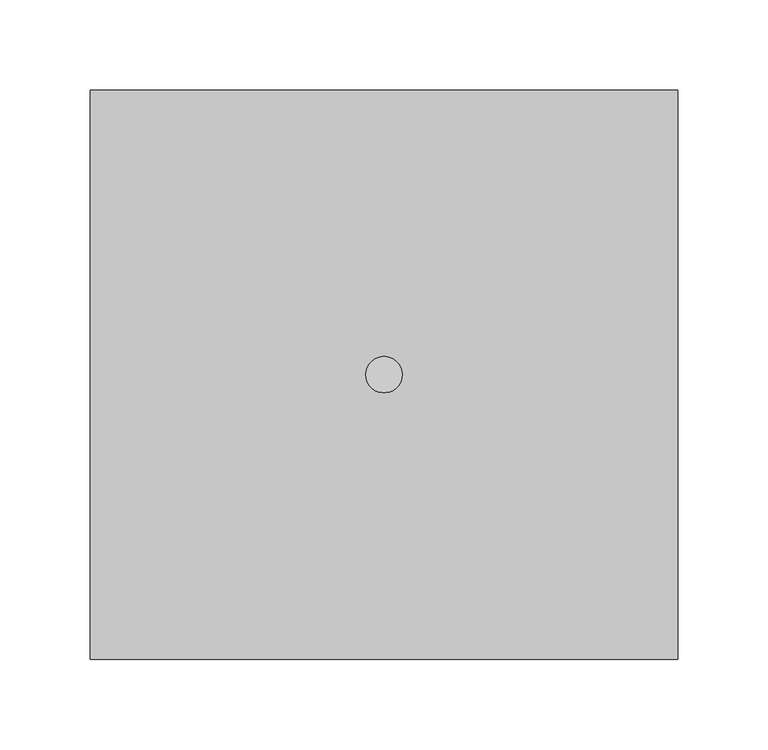
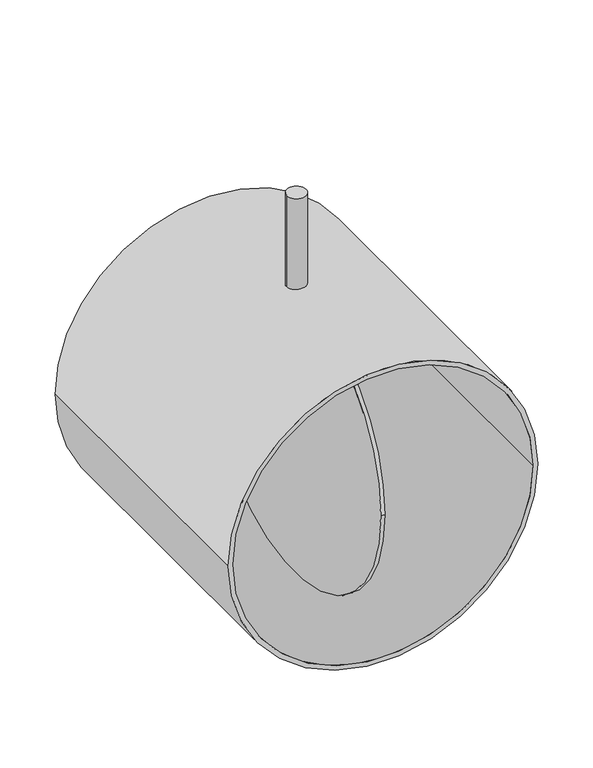
"""IFC4 building model written with IfcOpenShell, lengths in millimetres: proxy geometry, Заслонка регулирующая DFGR : DFGR 315."""

from ifc_helpers import new_model, si_unit, point, frame, origin, origin_2d, place, context, project, spatial, circle_curve, trimmed, segment, composite_curve, outline, extrude, source, transform, mapped, element, save


def mechanical_equipment_7cf25c75(model_context):
    return source(origin(), model_context, "Body", "SweptSolid", [
        extrude(outline(composite_curve([segment(trimmed(circle_curve(origin_2d(), 157.5), [point((-157.5, 0.0))], [point((157.5, 0.0))], False, "CARTESIAN"), True, "CONTINUOUS"), segment(trimmed(circle_curve(origin_2d(), 157.5), [point((157.5, 0.0))], [point((-157.5, 0.0))], False, "CARTESIAN"), True, "CONTINUOUS")], self_intersect=False)), frame((-2.0, 0.0, 0.0), z_axis=(1.0, 0.0, 0.0), x_axis=(0.0, 1.0, 0.0)), (0.0, 0.0, 1.0), 4.0),
        extrude(outline(composite_curve([segment(trimmed(circle_curve(origin_2d(), 10.0), [point((-10.0, 0.0))], [point((10.0, 0.0))], False, "CARTESIAN"), True, "CONTINUOUS"), segment(trimmed(circle_curve(origin_2d(), 10.0), [point((10.0, 0.0))], [point((-10.0, 0.0))], False, "CARTESIAN"), True, "CONTINUOUS")], self_intersect=False)), frame((0.0, 0.0, 160.0), z_axis=(0.0, 0.0, 1.0), x_axis=(1.0, 0.0, 0.0)), (0.0, 0.0, 1.0), 102.5),
        extrude(outline(composite_curve([segment(trimmed(circle_curve(origin_2d(), 162.5), [point((0.0, -162.5))], [point((0.0, 162.5))], False, "CARTESIAN"), True, "CONTINUOUS"), segment(trimmed(circle_curve(origin_2d(), 162.5), [point((0.0, 162.5))], [point((0.0, -162.5))], False, "CARTESIAN"), True, "CONTINUOUS")], self_intersect=False), holes=[composite_curve([segment(trimmed(circle_curve(origin_2d(), 157.5), [point((0.0, -157.5))], [point((0.0, 157.5))], True, "CARTESIAN"), True, "CONTINUOUS"), segment(trimmed(circle_curve(origin_2d(), 157.5), [point((0.0, 157.5))], [point((0.0, -157.5))], True, "CARTESIAN"), True, "CONTINUOUS")], self_intersect=False)]), frame((0.0, -157.5, 0.0), z_axis=(0.0, 1.0, 0.0), x_axis=(0.0, 0.0, 1.0)), (0.0, 0.0, 1.0), 315.0),
    ])


if __name__ == "__main__":
    model = new_model("IFC4")
    model_context = context("Model", 3, world=origin())
    ifc_project = project(units=[si_unit("LENGTHUNIT", "METRE", prefix="MILLI")], contexts=[model_context])
    site = spatial("IfcSite", under=ifc_project)
    building = spatial("IfcBuilding", under=site)
    placement = place(None, origin())
    mechanical_equipment_shape = mechanical_equipment_7cf25c75(model_context)
    element("IfcBuildingElementProxy", 1, Name="Заслонка регулирующая DFGR : DFGR 315", ObjectType="Заслонка регулирующая DFGR : DFGR 315", at=placement, inside=building, context=model_context, shape_type="MappedRepresentation", body=[
        mapped(mechanical_equipment_shape, transform((0.0, 0.0, 0.0), x_axis=(1.0, 0.0, 0.0), y_axis=(0.0, 1.0, 0.0), z_axis=(0.0, 0.0, 1.0))),
    ])
    save(model, "model.ifc")

# Revit data of these elements
# Type "Заслонка регулирующая DFGR : DFGR 315"
#   ADSK_Система_Имя [instance default] = ""
#   ADSK_Наименование краткое = "DFGR 315"
#   ADSK_Наименование [instance default] = "Регулирующая заслонка DFGR 315"
#   ADSK_Масса_Текст = "2.12"
#   ADSK_Марка = ""
#   ADSK_Код изделия = ""
#   ADSK_Завод-изготовитель = "WAER"
#   ADSK_Единица измерения = "шт."
#   ADSK_URL страницы изделия = ""
#   ADSK_URL документации изделия = ""
#   Высота = 160 mm
#   ADSK_Расход воздуха = 0 m³/h
#   ADSK_Размер_Длина_L = 315 mm
#   ADSK_Размер_Диаметр_D1 = 325 mm
#   ADSK_Размер_Диаметр_D = 315 mm
#   ADSK_Размер_Высота_H1 = 262.5 mm
#   ADSK_Размер_Высота_H = 425 mm
#   ADSK_Потеря давления воздуха = 0.0 Pa
#   ADSK_Масса = 2.12
#   ADSK_Количество [instance default] = 1
#   Default Elevation = 0
#   URL = ""
#   Cost = 0
